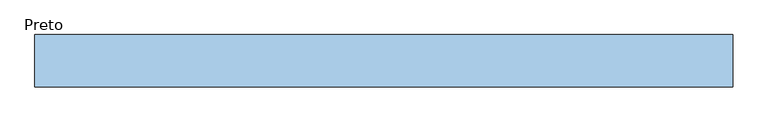
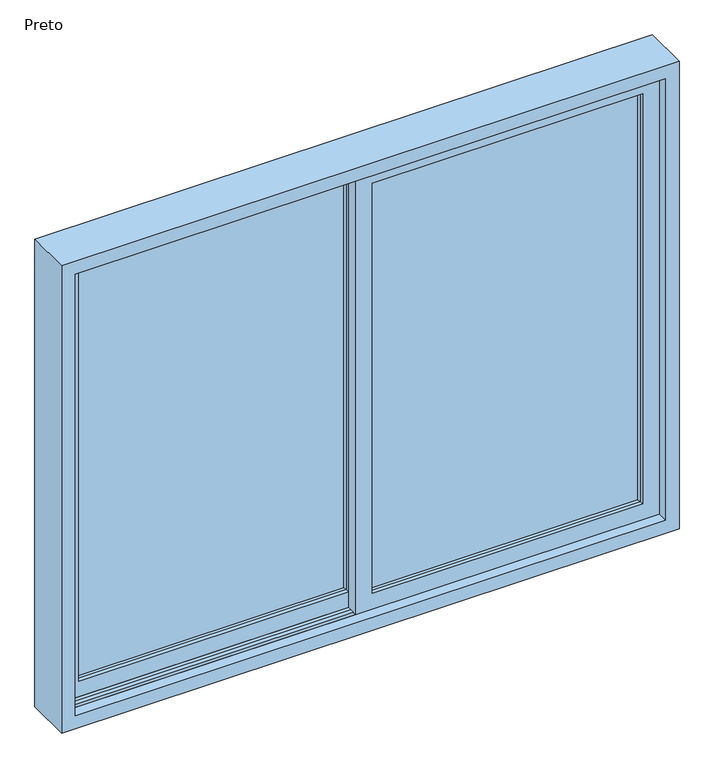
"""IFC4 building model written with IfcOpenShell, lengths in millimetres: window geometry, Blks_Cons Weiku_Janela de Correr 02 Folhas : Preto."""

from ifc_helpers import new_model, si_unit, frame, origin, place, context, project, spatial, polyline, outline, extrude, faceted_brep, source, transform, mapped, element, save


def preto_775ec973(model_context):
    return source(origin(), model_context, "Body", "SolidModel", [
        faceted_brep([(27.0, -13.0, 898.0), (27.0, -18.0, 898.0), (27.0, -18.0, 2302.0), (27.0, -13.0, 2302.0), (32.0, -18.0, 903.0), (32.0, -18.0, 2297.0), (902.0, -18.0, 2302.0), (902.0, -13.0, 2302.0), (897.0, -18.0, 2297.0), (902.0, -18.0, 898.0), (902.0, -13.0, 898.0), (897.0, -18.0, 903.0)], [[[0, 1, 2, 3]], [[4, 0, 3, 5]], [[3, 2, 6, 7]], [[5, 3, 7, 8]], [[7, 6, 9, 10]], [[8, 7, 10, 11]], [[1, 9, 6, 2], [5, 8, 11, 4]], [[10, 9, 1, 0]], [[11, 10, 0, 4]]]),
        faceted_brep([(902.0, -27.0, 898.0), (902.0, -22.0, 898.0), (902.0, -22.0, 2302.0), (902.0, -27.0, 2302.0), (27.0, -22.0, 2302.0), (27.0, -27.0, 2302.0), (27.0, -22.0, 898.0), (27.0, -27.0, 898.0), (897.0, -22.0, 2297.0), (32.0, -22.0, 2297.0), (32.0, -22.0, 903.0), (897.0, -22.0, 903.0)], [[[0, 1, 2, 3]], [[3, 2, 4, 5]], [[5, 4, 6, 7]], [[1, 6, 4, 2], [8, 9, 10, 11]], [[7, 6, 1, 0]], [[11, 0, 3, 8]], [[8, 3, 5, 9]], [[9, 5, 7, 10]], [[10, 7, 0, 11]]]),
        extrude(outline(polyline([(902.0, -22.0), (27.0, -22.0), (27.0, -18.0), (902.0, -18.0), (902.0, -22.0)])), frame((0.0, 0.0, 898.0), z_axis=(0.0, 0.0, 1.0), x_axis=(1.0, 0.0, 0.0)), (0.0, 0.0, 1.0), 1404.0),
        extrude(outline(polyline([(844.0, 956.0), (2356.0, 956.0), (2356.0, -27.0), (844.0, -27.0), (844.0, 956.0)]), holes=[polyline([(2302.0, 27.0), (2302.0, 902.0), (898.0, 902.0), (898.0, 27.0), (2302.0, 27.0)])]), frame((0.0, -40.0, 0.0), z_axis=(0.0, 1.0, 0.0), x_axis=(0.0, 0.0, 1.0)), (0.0, 0.0, 1.0), 40.0),
        faceted_brep([(-902.0, 27.0, 898.0), (-902.0, 22.0, 898.0), (-902.0, 22.0, 2302.0), (-902.0, 27.0, 2302.0), (-897.0, 22.0, 903.0), (-897.0, 22.0, 2297.0), (-27.0, 22.0, 2302.0), (-27.0, 27.0, 2302.0), (-32.0, 22.0, 2297.0), (-27.0, 22.0, 898.0), (-27.0, 27.0, 898.0), (-32.0, 22.0, 903.0)], [[[0, 1, 2, 3]], [[4, 0, 3, 5]], [[3, 2, 6, 7]], [[5, 3, 7, 8]], [[7, 6, 9, 10]], [[8, 7, 10, 11]], [[1, 9, 6, 2], [5, 8, 11, 4]], [[10, 9, 1, 0]], [[11, 10, 0, 4]]]),
        faceted_brep([(-27.0, 13.0, 898.0), (-27.0, 18.0, 898.0), (-27.0, 18.0, 2302.0), (-27.0, 13.0, 2302.0), (-902.0, 18.0, 2302.0), (-902.0, 13.0, 2302.0), (-902.0, 18.0, 898.0), (-902.0, 13.0, 898.0), (-32.0, 18.0, 2297.0), (-897.0, 18.0, 2297.0), (-897.0, 18.0, 903.0), (-32.0, 18.0, 903.0)], [[[0, 1, 2, 3]], [[3, 2, 4, 5]], [[5, 4, 6, 7]], [[1, 6, 4, 2], [8, 9, 10, 11]], [[7, 6, 1, 0]], [[11, 0, 3, 8]], [[8, 3, 5, 9]], [[9, 5, 7, 10]], [[10, 7, 0, 11]]]),
        extrude(outline(polyline([(-27.0, 18.0), (-902.0, 18.0), (-902.0, 22.0), (-27.0, 22.0), (-27.0, 18.0)])), frame((0.0, 0.0, 898.0), z_axis=(0.0, 0.0, 1.0), x_axis=(1.0, 0.0, 0.0)), (0.0, 0.0, 1.0), 1404.0),
        extrude(outline(polyline([(844.0, 27.0), (2356.0, 27.0), (2356.0, -956.0), (844.0, -956.0), (844.0, 27.0)]), holes=[polyline([(2302.0, -902.0), (2302.0, -27.0), (898.0, -27.0), (898.0, -902.0), (2302.0, -902.0)])]), frame((0.0, 0.0, 0.0), z_axis=(0.0, 1.0, 0.0), x_axis=(0.0, 0.0, 1.0)), (0.0, 0.0, 1.0), 40.0),
        faceted_brep([(956.0, 75.0, 844.0), (-956.0, 75.0, 844.0), (-956.0, 40.0, 844.0), (956.0, 40.0, 844.0), (-956.0, -75.0, 844.0), (956.0, -75.0, 844.0), (956.0, -40.0, 844.0), (-956.0, -40.0, 844.0), (-956.0, -13.0, 844.0), (-956.0, -27.0, 844.0), (956.0, -27.0, 844.0), (956.0, -13.0, 844.0), (-956.0, 27.0, 844.0), (-956.0, 13.0, 844.0), (956.0, 13.0, 844.0), (956.0, 27.0, 844.0), (1000.0, 75.0, 800.0), (-1000.0, 75.0, 800.0), (-1000.0, 75.0, 2400.0), (1000.0, 75.0, 2400.0), (956.0, 75.0, 2356.0), (-956.0, 75.0, 2356.0), (-956.0, 40.0, 2356.0), (-956.0, 40.0, 2366.0), (-956.0, 27.0, 2366.0), (-956.0, 27.0, 2356.0), (-956.0, 13.0, 2356.0), (-956.0, 13.0, 2366.0), (-956.0, -13.0, 2366.0), (-956.0, -13.0, 2356.0), (-956.0, -27.0, 2356.0), (-956.0, -27.0, 2366.0), (-956.0, -40.0, 2366.0), (-956.0, -40.0, 2356.0), (-956.0, -75.0, 2356.0), (-956.0, -40.0, 834.0), (-956.0, -27.0, 834.0), (-956.0, -13.0, 834.0), (-956.0, 13.0, 834.0), (-956.0, 27.0, 834.0), (-956.0, 40.0, 834.0), (956.0, 40.0, 834.0), (956.0, 27.0, 834.0), (956.0, 13.0, 834.0), (956.0, -13.0, 834.0), (956.0, -27.0, 834.0), (956.0, -40.0, 834.0), (956.0, -75.0, 2356.0), (956.0, -40.0, 2356.0), (956.0, -40.0, 2366.0), (956.0, -27.0, 2366.0), (956.0, -27.0, 2356.0), (956.0, -13.0, 2356.0), (956.0, -13.0, 2366.0), (956.0, 13.0, 2366.0), (956.0, 13.0, 2356.0), (956.0, 27.0, 2356.0), (956.0, 27.0, 2366.0), (956.0, 40.0, 2366.0), (956.0, 40.0, 2356.0), (-1000.0, -75.0, 800.0), (1000.0, -75.0, 800.0), (1000.0, -75.0, 2400.0), (-1000.0, -75.0, 2400.0)], [[[0, 1, 2, 3]], [[4, 5, 6, 7]], [[8, 9, 10, 11]], [[12, 13, 14, 15]], [[16, 17, 18, 19], [1, 0, 20, 21]], [[1, 21, 22, 23, 24, 25, 26, 27, 28, 29, 30, 31, 32, 33, 34, 4, 7, 35, 36, 9, 8, 37, 38, 13, 12, 39, 40, 2]], [[40, 41, 3, 2]], [[20, 0, 3, 41, 42, 15, 14, 43, 44, 11, 10, 45, 46, 6, 5, 47, 48, 49, 50, 51, 52, 53, 54, 55, 56, 57, 58, 59]], [[60, 61, 62, 63], [5, 4, 34, 47]], [[46, 35, 7, 6]], [[45, 10, 9, 36]], [[11, 44, 37, 8]], [[43, 14, 13, 38]], [[15, 42, 39, 12]], [[61, 16, 19, 62]], [[16, 61, 60, 17]], [[17, 60, 63, 18]], [[46, 45, 36, 35]], [[44, 43, 38, 37]], [[42, 41, 40, 39]], [[26, 25, 56, 55]], [[30, 29, 52, 51]], [[21, 20, 59, 22]], [[47, 34, 33, 48]], [[18, 63, 62, 19]], [[55, 54, 27, 26]], [[54, 53, 28, 27]], [[53, 52, 29, 28]], [[51, 50, 31, 30]], [[50, 49, 32, 31]], [[32, 49, 48, 33]], [[58, 23, 22, 59]], [[58, 57, 24, 23]], [[57, 56, 25, 24]]]),
    ])


if __name__ == "__main__":
    model = new_model("IFC4")
    model_context = context("Model", 3, world=origin())
    ifc_project = project(units=[si_unit("LENGTHUNIT", "METRE", prefix="MILLI")], contexts=[model_context])
    site = spatial("IfcSite", under=ifc_project)
    building = spatial("IfcBuilding", under=site)
    placement = place(None, origin())
    preto_shape = preto_775ec973(model_context)
    element("IfcWindow", 1, ObjectType="Blks_Cons Weiku_Janela de Correr 02 Folhas : Preto", at=placement, inside=building, context=model_context, shape_type="MappedRepresentation", body=[
        mapped(preto_shape, transform((0.0, 0.0, 0.0), x_axis=(1.0, 0.0, 0.0), y_axis=(0.0, 1.0, 0.0), z_axis=(0.0, 0.0, 1.0))),
    ])
    save(model, "model.ifc")

# Revit data of these elements
# Type "Blks_Cons Weiku_Janela de Correr 02 Folhas : Preto"
#   Type Mark = "J26"
#   Type Comments = "Janela de Correr 02 Folhas"
#   Manufacturer = "Weiku"
#   Created By / Criado Por / Creado por = "Blocks"
#   Author URL = "https://BlocksRvt.com/"
#   Author Contact = "info@blocksrvt.com"
#   Assembly Code = "Cons"
#   c [instance default] = 250 mm
#   b [instance default] = 912 mm
#   a [instance default] = 983 mm
#   Rough Width [instance default] = 2000 mm
#   Width [instance default] = 1912 mm
#   Espessura Folha [instance default] = 40 mm
#   Rough Height [instance default] = 1000 mm
#   Height [instance default] = 912 mm
#   Abertura Janela Equerda [instance default] = 0 mm
#   Abertura Janela Direita [instance default] = 0 mm
#   Vidro = .vidro_growarq
#   Vedação = Blks - Rubber - Black
#   Janela = Blks - Plastic - Black - Glazed
#   Wall Closure = (empty or 0)
# Element 1 (IfcWindow, "Blks_Cons Weiku_Janela de Correr 02 Folhas : Preto")
#   b = 1512 mm
#   Rough Height = 1600 mm
#   Height = 1512 mm
#   Materials on its faces: "Blks - Plastic - Black - Glazed", "Blks - Rubber - Black", ".vidro_growarq"
# Materials
#   ".vidro_growarq": class "Vidro", colour RGB 200 215 215, transparency 0.6, Description = "Vidroverde", Cost = 0
#   "Blks - Rubber - Black": class "Paint/Coating", colour RGB 38 38 38, transparency 0, Cost = 0
#   "Blks - Plastic - Black - Glazed": class "Plastic", colour RGB 25 25 25, transparency 0, Cost = 0
